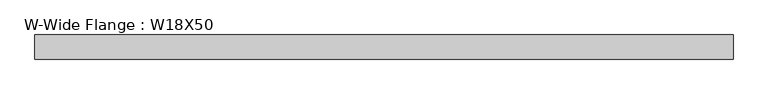
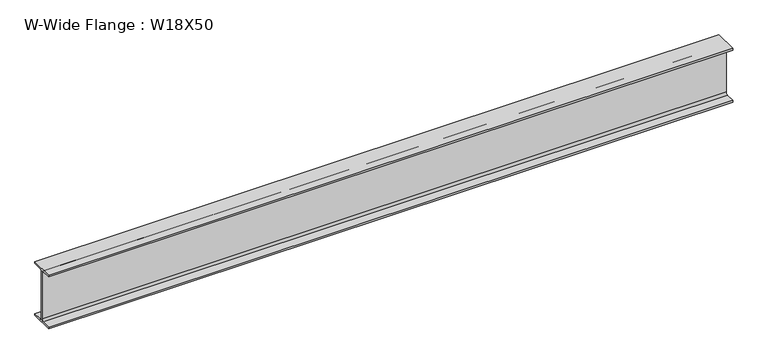
"""IFC4 building model written with IfcOpenShell, lengths in millimetres: beam geometry, W-Wide Flange : W18X50."""

from ifc_helpers import new_model, si_unit, point, frame, frame_2d, origin, place, context, project, spatial, polyline, circle_curve, trimmed, segment, composite_curve, outline, extrude, source, transform, mapped, element, save


def w_wide_flange_w18x50_f803f88f(model_context):
    return source(origin(), model_context, "Body", "SweptSolid", [
        extrude(outline(composite_curve([segment(polyline([(95.25, -214.122), (95.25, -228.6), (-95.25, -228.6), (-95.25, -214.122), (-21.7805, -214.122)]), True, "CONTINUOUS"), segment(trimmed(circle_curve(frame_2d((-21.7805, -196.85)), 17.272), [point((-21.7805, -214.122))], [point((-4.5085, -196.85))], True, "CARTESIAN"), True, "CONTINUOUS"), segment(polyline([(-4.5085, -196.85), (-4.5085, 196.85)]), True, "CONTINUOUS"), segment(trimmed(circle_curve(frame_2d((-21.7805, 196.85)), 17.272), [point((-4.5085, 196.85))], [point((-21.7805, 214.122))], True, "CARTESIAN"), True, "CONTINUOUS"), segment(polyline([(-21.7805, 214.122), (-95.25, 214.122), (-95.25, 228.6), (95.25, 228.6), (95.25, 214.122), (21.7805, 214.122)]), True, "CONTINUOUS"), segment(trimmed(circle_curve(frame_2d((21.7805, 196.85)), 17.272), [point((21.7805, 214.122))], [point((4.5085, 196.85))], True, "CARTESIAN"), True, "CONTINUOUS"), segment(polyline([(4.5085, 196.85), (4.5085, -196.85)]), True, "CONTINUOUS"), segment(trimmed(circle_curve(frame_2d((21.7805, -196.85)), 17.272), [point((4.5085, -196.85))], [point((21.7805, -214.122))], True, "CARTESIAN"), True, "CONTINUOUS"), segment(polyline([(21.7805, -214.122), (95.25, -214.122)]), True, "CONTINUOUS")], self_intersect=False)), frame((-2755.9, 0.0, 0.0), z_axis=(1.0, 0.0, 0.0), x_axis=(0.0, 1.0, 0.0)), (0.0, 0.0, 1.0), 5511.8),
    ])


if __name__ == "__main__":
    model = new_model("IFC4")
    model_context = context("Model", 3, world=origin())
    ifc_project = project(units=[si_unit("LENGTHUNIT", "METRE", prefix="MILLI")], contexts=[model_context])
    site = spatial("IfcSite", under=ifc_project)
    building = spatial("IfcBuilding", under=site)
    placement = place(None, origin())
    w_wide_flange_w18x50_shape = w_wide_flange_w18x50_f803f88f(model_context)
    element("IfcBeam", 1, ObjectType="W-Wide Flange : W18X50", at=placement, inside=building, context=model_context, shape_type="MappedRepresentation", body=[
        mapped(w_wide_flange_w18x50_shape, transform((0.0, 0.0, 0.0), x_axis=(1.0, 0.0, 0.0), y_axis=(0.0, 1.0, 0.0), z_axis=(0.0, 0.0, 1.0))),
    ])
    save(model, "model.ifc")

# Revit data of these elements
# Type "W-Wide Flange : W18X50"
#   Assembly Code = "B10"
#   W = 50
#   Length [instance default] = 5' - 0"
#   bf = 0' - 7 1/2"
#   d = 1' - 6"
#   k = 0' - 1 1/4"
#   k2 = 0' - 0.68"
#   tf = 0' - 0.57"
#   tw = 0' - 0.355"
#   A = 0.102083 SF
#   Structural Material [instance default] = Steel ASTM A992
# Element 1 (IfcBeam, "W-Wide Flange : W18X50")
#   Materials on its faces: "Steel ASTM A992"
# Materials
#   "Steel ASTM A992": class "Metal", colour RGB 199 199 199, transparency 0, Description = "Structural steel 50ksi", Cost = 0
